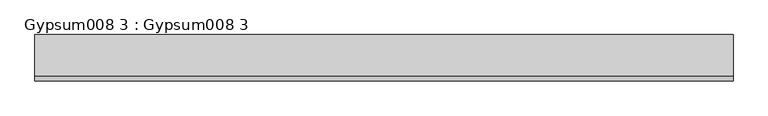
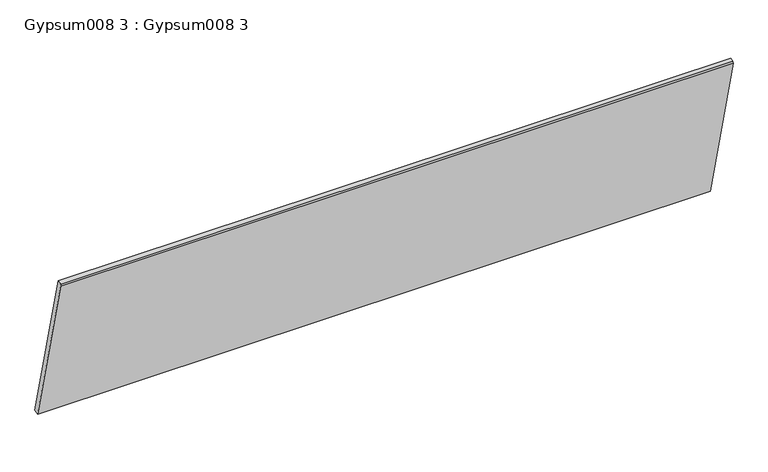
"""IFC4 building model written with IfcOpenShell, lengths in millimetres: proxy geometry, Gypsum008 3 : Gypsum008 3."""

from ifc_helpers import new_model, si_unit, frame, origin, place, context, project, spatial, polyline, outline, extrude, source, transform, mapped, element, save


def gypsum008_3_gypsum008_3_d0d3208e(model_context):
    return source(origin(), model_context, "Body", "SweptSolid", [
        extrude(outline(polyline([(9752.047493, 43222.0071182), (9737.9368073, 43218.4770293), (9619.3816911, 43692.3727377), (9619.9854477, 43698.7661533), (9632.0226951, 43701.7775274), (9752.047493, 43222.0071182)])), frame((3694.2883192, 0.0, 0.0), z_axis=(1.0, 0.0, 0.0), x_axis=(0.0, 1.0, 0.0)), (0.0, 0.0, 1.0), 2000.0),
    ])


if __name__ == "__main__":
    model = new_model("IFC4")
    model_context = context("Model", 3, world=origin())
    ifc_project = project(units=[si_unit("LENGTHUNIT", "METRE", prefix="MILLI")], contexts=[model_context])
    site = spatial("IfcSite", under=ifc_project)
    building = spatial("IfcBuilding", under=site)
    placement = place(None, origin())
    gypsum008_3_gypsum008_3_shape = gypsum008_3_gypsum008_3_d0d3208e(model_context)
    element("IfcBuildingElementProxy", 1, Name="Gypsum008 3 : Gypsum008 3", ObjectType="Gypsum008 3 : Gypsum008 3", at=placement, inside=building, context=model_context, shape_type="MappedRepresentation", body=[
        mapped(gypsum008_3_gypsum008_3_shape, transform((0.0, 0.0, 0.0), x_axis=(1.0, 0.0, 0.0), y_axis=(0.0, 1.0, 0.0), z_axis=(0.0, 0.0, 1.0))),
    ])
    save(model, "model.ifc")

# Revit data of these elements
# Type "Gypsum008 3 : Gypsum008 3"
#   NameOverride = "Gypsum008"
# Element 1 (IfcBuildingElementProxy, "Gypsum008 3 : Gypsum008 3")
#   Materials on its faces: "5/8\"  GYPSUM BOARD"
# Materials
#   "5/8\"  GYPSUM BOARD": class "Unassigned", colour RGB 255 255 255, transparency 0, Cost = 0
